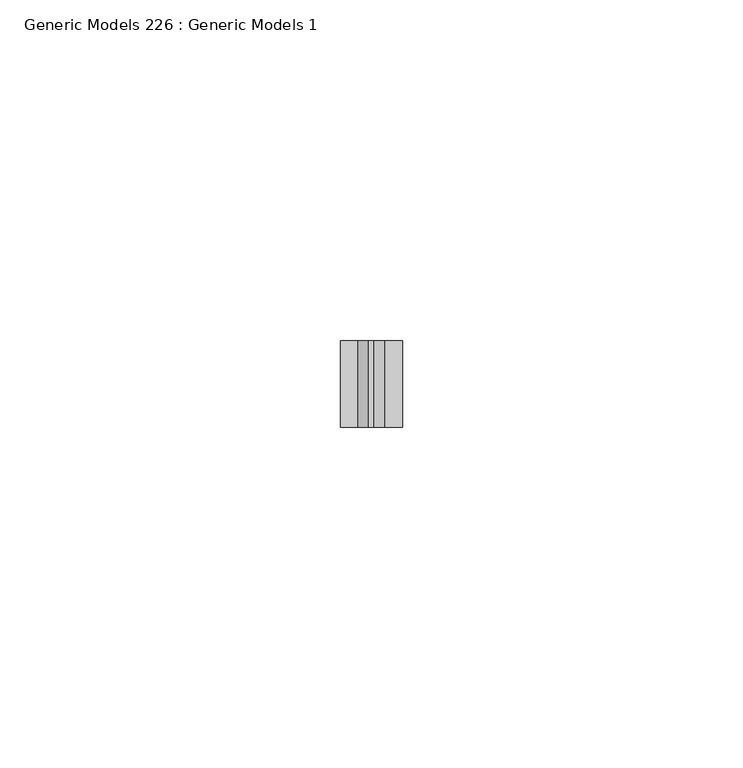
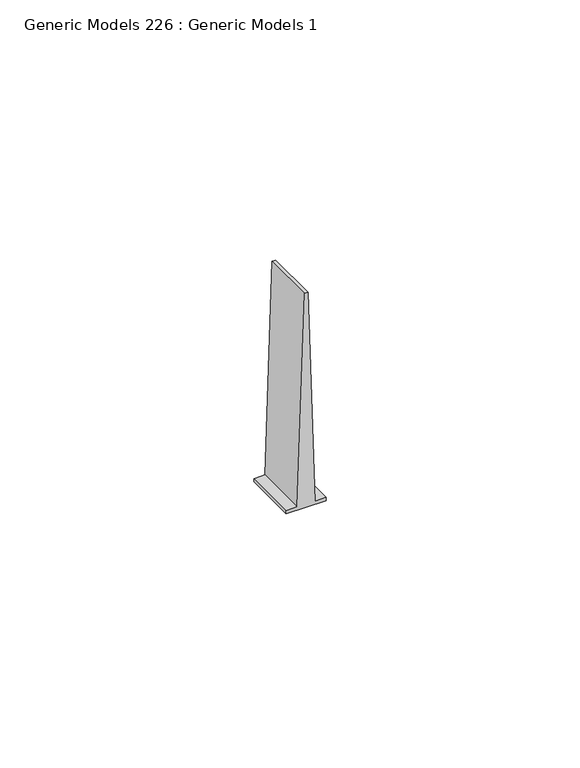
"""IFC4 building model written with IfcOpenShell, lengths in millimetres: proxy geometry, Generic Models 226 : Generic Models 1."""

from ifc_helpers import new_model, si_unit, frame, origin, place, context, project, spatial, polyline, outline, extrude, source, transform, mapped, element, save


def generic_models_226_generic_models_1_7dc37832(model_context):
    return source(origin(), model_context, "Body", "SweptSolid", [
        extrude(outline(polyline([(5263.35625, 49733.4159), (5263.35625, 49742.5091), (5264.15, 49742.5091), (5264.15, 49739.9592364), (5314.95, 49738.3618473), (5314.95, 49737.5631527), (5264.15, 49735.9657636), (5264.15, 49733.4159), (5263.35625, 49733.4159)])), frame((0.0, 565.15, 0.0), z_axis=(0.0, 1.0, 0.0), x_axis=(0.0, 0.0, 1.0)), (0.0, 0.0, 1.0), 12.7),
    ])


if __name__ == "__main__":
    model = new_model("IFC4")
    model_context = context("Model", 3, world=origin())
    ifc_project = project(units=[si_unit("LENGTHUNIT", "METRE", prefix="MILLI")], contexts=[model_context])
    site = spatial("IfcSite", under=ifc_project)
    building = spatial("IfcBuilding", under=site)
    placement = place(None, origin())
    generic_models_226_generic_models_1_shape = generic_models_226_generic_models_1_7dc37832(model_context)
    element("IfcBuildingElementProxy", 1, Name="Generic Models 226 : Generic Models 1", ObjectType="Generic Models 226 : Generic Models 1", at=placement, inside=building, context=model_context, shape_type="MappedRepresentation", body=[
        mapped(generic_models_226_generic_models_1_shape, transform((0.0, 0.0, 0.0), x_axis=(1.0, 0.0, 0.0), y_axis=(0.0, 1.0, 0.0), z_axis=(0.0, 0.0, 1.0))),
    ])
    save(model, "model.ifc")

# Revit data of these elements
# Element 1 (IfcBuildingElementProxy, "Generic Models 226 : Generic Models 1")
#   Materials on its faces: "METAL RUNNER CHANNEL; FASTEN @ 24\" O.C."
# Materials
#   "METAL RUNNER CHANNEL; FASTEN @ 24\" O.C.": class "Unassigned", colour RGB 210 209 208, transparency 0, Keynote = "M05121300.02", Cost = 0
